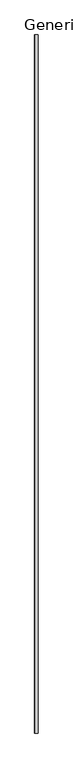
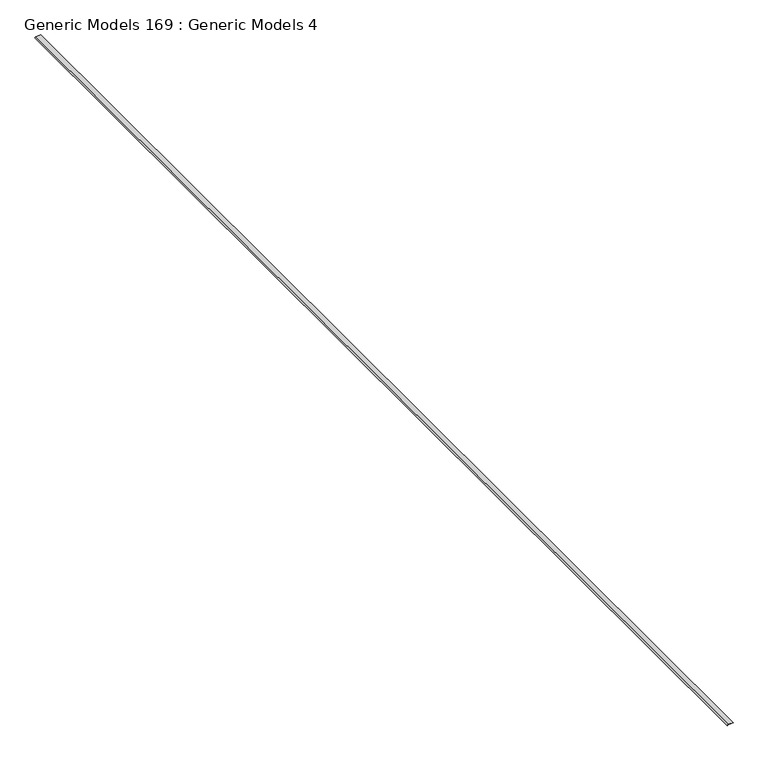
"""IFC4 building model written with IfcOpenShell, lengths in millimetres: proxy geometry, Generic Models 169 : Generic Models 4."""

from ifc_helpers import new_model, si_unit, frame, origin, place, context, project, spatial, polyline, outline, extrude, source, transform, mapped, element, save


def generic_models_169_generic_models_4_a8ea786d(model_context):
    return source(origin(), model_context, "Body", "SweptSolid", [
        extrude(outline(polyline([(122947.2593368, -10290.974673), (122947.2593368, -10238.6940484), (122948.8468368, -10238.6940484), (122948.8468368, -10291.8010732), (122937.7666585, -10299.5594976), (122936.8561059, -10298.2590937), (122947.2593368, -10290.974673)])), frame((0.0, -5493.3230338, 0.0), z_axis=(0.0, 1.0, 0.0), x_axis=(0.0, 0.0, 1.0)), (0.0, 0.0, 1.0), 12547.6),
    ])


if __name__ == "__main__":
    model = new_model("IFC4")
    model_context = context("Model", 3, world=origin())
    ifc_project = project(units=[si_unit("LENGTHUNIT", "METRE", prefix="MILLI")], contexts=[model_context])
    site = spatial("IfcSite", under=ifc_project)
    building = spatial("IfcBuilding", under=site)
    placement = place(None, origin())
    generic_models_169_generic_models_4_shape = generic_models_169_generic_models_4_a8ea786d(model_context)
    element("IfcBuildingElementProxy", 1, Name="Generic Models 169 : Generic Models 4", ObjectType="Generic Models 169 : Generic Models 4", at=placement, inside=building, context=model_context, shape_type="MappedRepresentation", body=[
        mapped(generic_models_169_generic_models_4_shape, transform((0.0, 0.0, 0.0), x_axis=(1.0, 0.0, 0.0), y_axis=(0.0, 1.0, 0.0), z_axis=(0.0, 0.0, 1.0))),
    ])
    save(model, "model.ifc")

# Revit data of these elements
# Element 1 (IfcBuildingElementProxy, "Generic Models 169 : Generic Models 4")
#   Materials on its faces: "_CONT. 16 GA. COPPER DRIP FLASHING"
# Materials
#   "_CONT. 16 GA. COPPER DRIP FLASHING": class "Metal", colour RGB 199 199 199, transparency 0, Description = "Structural steel 50ksi", Cost = 0
